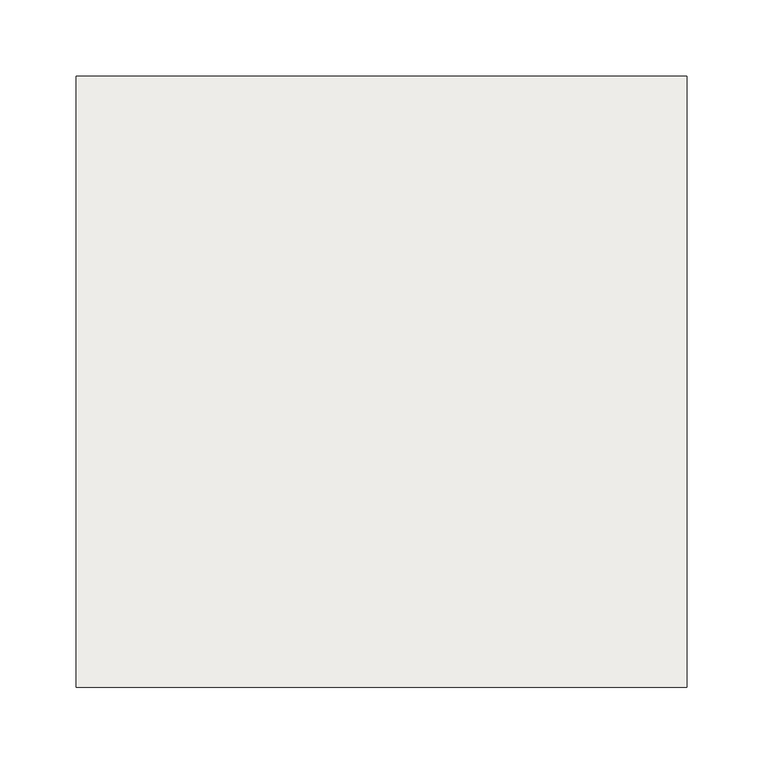
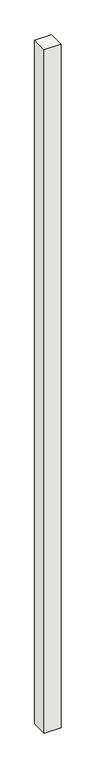
"""IFC4 building model written with IfcOpenShell, lengths in millimetres: slab geometry, NLRS_17_SFO_TLB_funderingspaal geheid beton prefab-AV-MMBPC_gen_rsf : heipaal beton prefab_gen__bxh 400x400."""

from ifc_helpers import new_model, si_unit, frame, origin, place, context, project, spatial, polyline, outline, extrude, source, transform, mapped, element, save


def slab_73a1868d(model_context):
    return source(origin(), model_context, "Body", "SweptSolid", [
        extrude(outline(polyline([(200.0, -200.0), (-200.0, -200.0), (-200.0, 200.0), (200.0, 200.0), (200.0, -200.0)])), frame((0.0, 0.0, -20000.0), z_axis=(0.0, 0.0, 1.0), x_axis=(1.0, 0.0, 0.0)), (0.0, 0.0, 1.0), 17400.0),
    ])


if __name__ == "__main__":
    model = new_model("IFC4")
    model_context = context("Model", 3, world=origin())
    ifc_project = project(units=[si_unit("LENGTHUNIT", "METRE", prefix="MILLI")], contexts=[model_context])
    site = spatial("IfcSite", under=ifc_project)
    building = spatial("IfcBuilding", under=site)
    placement = place(None, origin())
    slab_shape = slab_73a1868d(model_context)
    element("IfcSlab", 1, ObjectType="NLRS_17_SFO_TLB_funderingspaal geheid beton prefab-AV-MMBPC_gen_rsf : heipaal beton prefab_gen__bxh 400x400", at=placement, inside=building, context=model_context, shape_type="MappedRepresentation", body=[
        mapped(slab_shape, transform((0.0, 0.0, 0.0), x_axis=(1.0, 0.0, 0.0), y_axis=(0.0, 1.0, 0.0), z_axis=(0.0, 0.0, 1.0))),
    ])
    save(model, "model.ifc")

# Revit data of these elements
# Type "NLRS_17_SFO_TLB_funderingspaal geheid beton prefab-AV-MMBPC_gen_rsf : heipaal beton prefab_gen__bxh 400x400"
#   Export Type to IFC As = "IfcPile"
#   Type IfcGUID = "10$Kfo5uPCAOPJEOo5LE_W"
#   Type Comments = "prefab heipaal 400x400"
#   Model = " "
#   Manufacturer = " "
#   Description = "prefab heipaal 400x400"
#   Assembly Code = "17.21"
#   Width = 400 mm
#   Slanted Angle [instance default] = 0.00°
#   NLRS_S_draagvermogen_trek [instance default] = 0.00 kN
#   NLRS_S_draagvermogen_druk [instance default] = 0.00 kN
#   NLRS_C_lengte [instance default] = 1660 mm
#   NLRS_C_hoogte = 400 mm
#   NLRS_C_breedte = 400 mm
#   Height [instance default] = 1660 mm
#   Length [instance default] = 1660 mm
#   Angle [instance default] = 0.00°
#   Slanted [instance default] = 0
#   Structural Material = NLRS_f2_beton prefab_gen_rsf
#   Keynote = ""
# Element 1 (IfcSlab, "NLRS_17_SFO_TLB_funderingspaal geheid beton prefab-AV-MMBPC_gen_rsf : heipaal beton prefab_gen__bxh 400x400")
#   NLRS_C_lengte = 17400 mm
#   Height = 17400 mm
#   Length = 17400 mm
#   Materials on its faces: "NLRS_f2_beton prefab_gen_rsf"
# Materials
#   "NLRS_f2_beton prefab_gen_rsf": class "F - Niet gebakken kunststeen", colour RGB 129 133 118, transparency 0, Keynote = "f2", Manufacturer = "Revit Standards Foundation", URL = "www.revitstandards.org", Description = "beton prefab", Cost = 0
